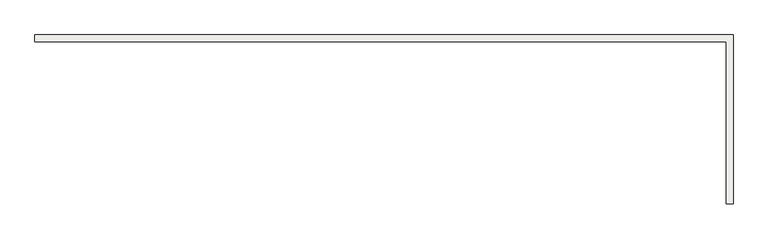
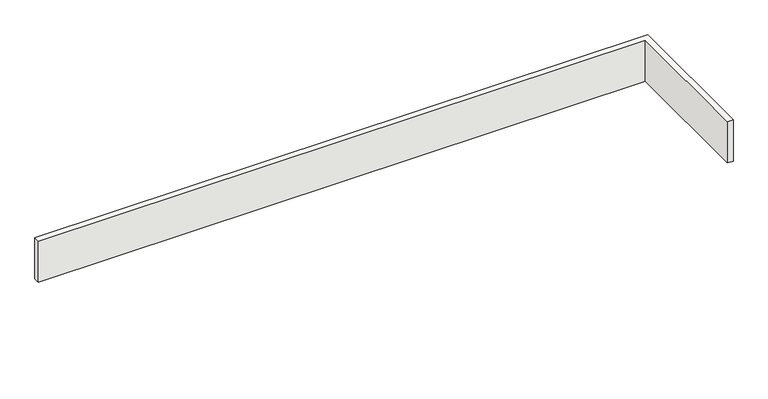
"""IFC4 building model written with IfcOpenShell, lengths in millimetres: slab geometry, RODAPÉ BANCADA CHURRASQUEIRA : RODAPÉ BANCADA CHURRASQUEIRA."""

from ifc_helpers import new_model, si_unit, frame, origin, place, context, project, spatial, polyline, outline, extrude, source, transform, mapped, element, save


def slab_7a94a420(model_context):
    return source(origin(), model_context, "Body", "SweptSolid", [
        extrude(outline(polyline([(6741.1852269, -4474.440479), (6741.1852269, -4454.440479), (8851.1852269, -4454.440479), (8851.1852269, -4964.440479), (8831.1852269, -4964.440479), (8831.1852269, -4474.440479), (6741.1852269, -4474.440479)])), frame((0.0, 0.0, 400.0), z_axis=(0.0, 0.0, 1.0), x_axis=(1.0, 0.0, 0.0)), (0.0, 0.0, 1.0), 150.0),
    ])


if __name__ == "__main__":
    model = new_model("IFC4")
    model_context = context("Model", 3, world=origin())
    ifc_project = project(units=[si_unit("LENGTHUNIT", "METRE", prefix="MILLI")], contexts=[model_context])
    site = spatial("IfcSite", under=ifc_project)
    building = spatial("IfcBuilding", under=site)
    placement = place(None, origin())
    slab_shape = slab_7a94a420(model_context)
    element("IfcSlab", 1, ObjectType="RODAPÉ BANCADA CHURRASQUEIRA : RODAPÉ BANCADA CHURRASQUEIRA", at=placement, inside=building, context=model_context, shape_type="MappedRepresentation", body=[
        mapped(slab_shape, transform((0.0, 0.0, 0.0), x_axis=(1.0, 0.0, 0.0), y_axis=(0.0, 1.0, 0.0), z_axis=(0.0, 0.0, 1.0))),
    ])
    save(model, "model.ifc")

# Revit data of these elements
# Element 1 (IfcSlab, "RODAPÉ BANCADA CHURRASQUEIRA : RODAPÉ BANCADA CHURRASQUEIRA")
#   Materials on its faces: ".GRANITO_BRANCO_ITAUNAS"
# Materials
#   ".GRANITO_BRANCO_ITAUNAS": class ".CC_PEDRA REVEST.", colour RGB 202 195 174, transparency 0, Description = "Revestimento em granito", Cost = 0
